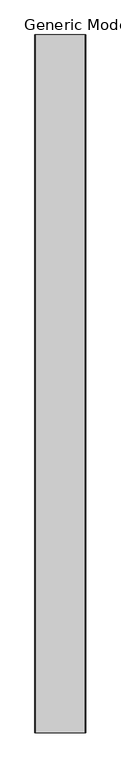
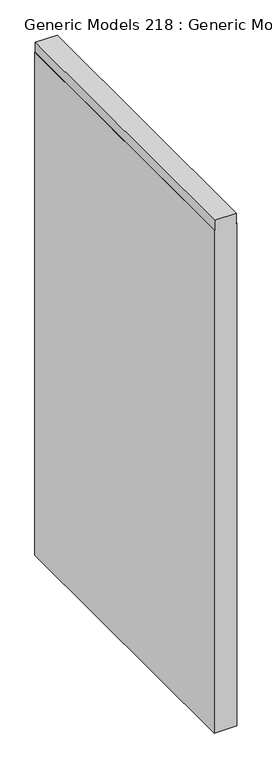
"""IFC4 building model written with IfcOpenShell, lengths in millimetres: proxy geometry, Generic Models 218 : Generic Models 208."""

from ifc_helpers import new_model, si_unit, frame, origin, place, context, project, spatial, polyline, outline, extrude, source, transform, mapped, element, save


def generic_models_218_generic_models_208_f75aa3c8(model_context):
    return source(origin(), model_context, "Body", "SweptSolid", [
        extrude(outline(polyline([(2088.753125, 55769.6454676), (2130.028125, 55769.6454676), (2130.028125, 55683.9204676), (2088.753125, 55683.9204676), (2088.753125, 55682.3329676), (1.5875, 55682.3329676), (1.5875, 55771.2329676), (2088.753125, 55771.2329676), (2088.753125, 55769.6454676)])), frame((0.0, -228.7033818, 0.0), z_axis=(0.0, 1.0, 0.0), x_axis=(0.0, 0.0, 1.0)), (0.0, 0.0, 1.0), 1219.2),
    ])


if __name__ == "__main__":
    model = new_model("IFC4")
    model_context = context("Model", 3, world=origin())
    ifc_project = project(units=[si_unit("LENGTHUNIT", "METRE", prefix="MILLI")], contexts=[model_context])
    site = spatial("IfcSite", under=ifc_project)
    building = spatial("IfcBuilding", under=site)
    placement = place(None, origin())
    generic_models_218_generic_models_208_shape = generic_models_218_generic_models_208_f75aa3c8(model_context)
    element("IfcBuildingElementProxy", 1, Name="Generic Models 218 : Generic Models 208", ObjectType="Generic Models 218 : Generic Models 208", at=placement, inside=building, context=model_context, shape_type="MappedRepresentation", body=[
        mapped(generic_models_218_generic_models_208_shape, transform((0.0, 0.0, 0.0), x_axis=(1.0, 0.0, 0.0), y_axis=(0.0, 1.0, 0.0), z_axis=(0.0, 0.0, 1.0))),
    ])
    save(model, "model.ifc")

# Revit data of these elements
# Element 1 (IfcBuildingElementProxy, "Generic Models 218 : Generic Models 208")
#   Materials on its faces: "METAL STUDS"
# Materials
#   "METAL STUDS": class "Unassigned", colour RGB 210 209 208, transparency 0, Keynote = "M05121300.02", Cost = 0
